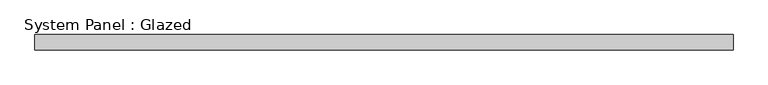
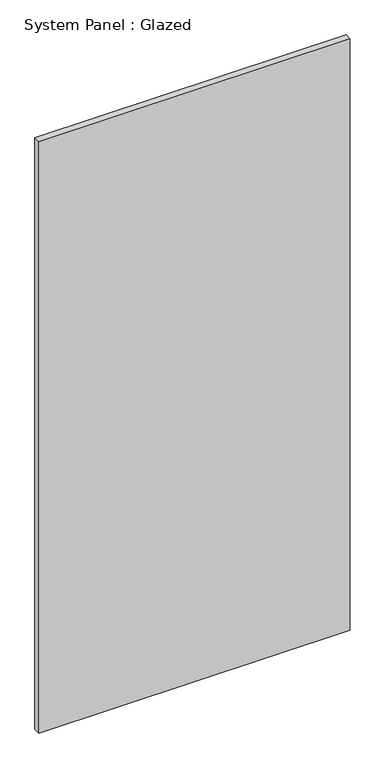
"""IFC4 building model written with IfcOpenShell, lengths in millimetres: plate geometry, System Panel : Glazed."""

from ifc_helpers import new_model, si_unit, origin, origin_with_axes, place, context, project, spatial, polyline, outline, extrude, source, transform, mapped, element, save


def system_panel_glazed_75b9e84a(model_context):
    return source(origin(), model_context, "Body", "SweptSolid", [
        extrude(outline(polyline([(583.1416667, 19.05), (-583.1416667, 19.05), (-583.1416667, 44.45), (583.1416667, 44.45), (583.1416667, 19.05)])), origin_with_axes(), (0.0, 0.0, 1.0), 2343.15),
    ])


if __name__ == "__main__":
    model = new_model("IFC4")
    model_context = context("Model", 3, world=origin())
    ifc_project = project(units=[si_unit("LENGTHUNIT", "METRE", prefix="MILLI")], contexts=[model_context])
    site = spatial("IfcSite", under=ifc_project)
    building = spatial("IfcBuilding", under=site)
    placement = place(None, origin())
    system_panel_glazed_shape = system_panel_glazed_75b9e84a(model_context)
    element("IfcPlate", 1, ObjectType="System Panel : Glazed", at=placement, inside=building, context=model_context, shape_type="MappedRepresentation", body=[
        mapped(system_panel_glazed_shape, transform((0.0, 0.0, 0.0), x_axis=(1.0, 0.0, 0.0), y_axis=(0.0, 1.0, 0.0), z_axis=(0.0, 0.0, 1.0))),
    ])
    save(model, "model.ifc")

# Revit data of these elements
# Element 1 (IfcPlate, "System Panel : Glazed")
#   Materials on its faces: "Glass"
# Materials
#   "Glass": class "Glass", colour RGB 218 227 224, transparency 0.85, Description = "Soda Lime Glass", Cost = 0
